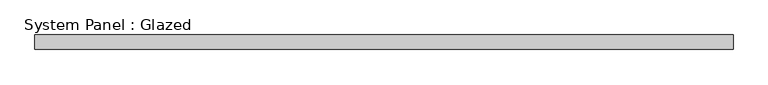
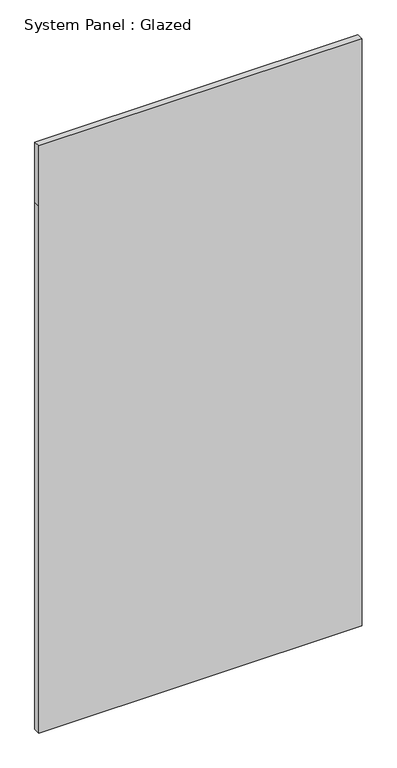
"""IFC4 building model written with IfcOpenShell, lengths in millimetres: plate geometry, System Panel : Glazed."""

from ifc_helpers import new_model, si_unit, frame, origin, place, context, project, spatial, polyline, outline, extrude, source, transform, mapped, element, save


def system_panel_glazed_b962cb7b(model_context):
    return source(origin(), model_context, "Body", "SweptSolid", [
        extrude(outline(polyline([(0.0, -610.2825643), (0.0, 610.2825643), (2101.85, 610.2825643), (2343.15, 610.2825643), (2343.15, -610.2825643), (2101.85, -610.2825643), (0.0, -610.2825643)])), frame((0.0, 19.05, 0.0), z_axis=(0.0, 1.0, 0.0), x_axis=(0.0, 0.0, 1.0)), (0.0, 0.0, 1.0), 25.4),
    ])


if __name__ == "__main__":
    model = new_model("IFC4")
    model_context = context("Model", 3, world=origin())
    ifc_project = project(units=[si_unit("LENGTHUNIT", "METRE", prefix="MILLI")], contexts=[model_context])
    site = spatial("IfcSite", under=ifc_project)
    building = spatial("IfcBuilding", under=site)
    placement = place(None, origin())
    system_panel_glazed_shape = system_panel_glazed_b962cb7b(model_context)
    element("IfcPlate", 1, ObjectType="System Panel : Glazed", at=placement, inside=building, context=model_context, shape_type="MappedRepresentation", body=[
        mapped(system_panel_glazed_shape, transform((0.0, 0.0, 0.0), x_axis=(1.0, 0.0, 0.0), y_axis=(0.0, 1.0, 0.0), z_axis=(0.0, 0.0, 1.0))),
    ])
    save(model, "model.ifc")

# Revit data of these elements
# Element 1 (IfcPlate, "System Panel : Glazed")
#   Materials on its faces: "Glass"
# Materials
#   "Glass": class "Glass", colour RGB 0 128 192, transparency 0.75
